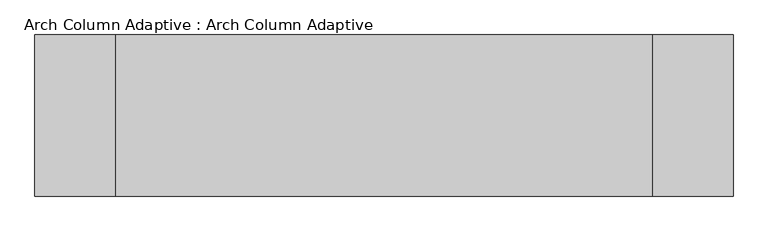
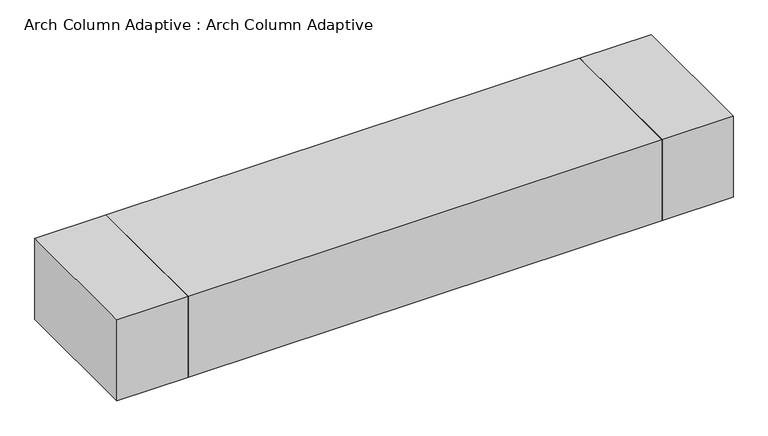
"""IFC4 building model written with IfcOpenShell, lengths in millimetres: proxy geometry, Arch Column Adaptive : Arch Column Adaptive."""

from ifc_helpers import new_model, si_unit, frame, origin, place, context, project, spatial, polyline, outline, extrude, source, transform, mapped, element, save


def arch_column_adaptive_arch_column_adaptive_6fcdb71c(model_context):
    return source(origin(), model_context, "Body", "SweptSolid", [
        extrude(outline(polyline([(5000.0, -1500.0), (5000.0, 1500.0), (6500.0, 1500.0), (6500.0, -1500.0), (5000.0, -1500.0)])), frame((0.0, 0.0, 23611.4), z_axis=(0.0, 0.0, 1.0), x_axis=(1.0, 0.0, 0.0)), (0.0, 0.0, 1.0), 1800.0),
        extrude(outline(polyline([(-5000.0, 1500.0), (-5000.0, -1500.0), (-6500.0, -1500.0), (-6500.0, 1500.0), (-5000.0, 1500.0)])), frame((0.0, 0.0, 23611.4), z_axis=(0.0, 0.0, 1.0), x_axis=(1.0, 0.0, 0.0)), (0.0, 0.0, 1.0), 1800.0),
        extrude(outline(polyline([(-5000.0, -1500.0), (-5000.0, 1500.0), (5000.0, 1500.0), (5000.0, -1500.0), (-5000.0, -1500.0)])), frame((0.0, 0.0, 23611.4), z_axis=(0.0, 0.0, 1.0), x_axis=(1.0, 0.0, 0.0)), (0.0, 0.0, 1.0), 1800.0),
    ])


if __name__ == "__main__":
    model = new_model("IFC4")
    model_context = context("Model", 3, world=origin())
    ifc_project = project(units=[si_unit("LENGTHUNIT", "METRE", prefix="MILLI")], contexts=[model_context])
    site = spatial("IfcSite", under=ifc_project)
    building = spatial("IfcBuilding", under=site)
    placement = place(None, origin())
    arch_column_adaptive_arch_column_adaptive_shape = arch_column_adaptive_arch_column_adaptive_6fcdb71c(model_context)
    element("IfcBuildingElementProxy", 1, Name="Arch Column Adaptive : Arch Column Adaptive", ObjectType="Arch Column Adaptive : Arch Column Adaptive", at=placement, inside=building, context=model_context, shape_type="MappedRepresentation", body=[
        mapped(arch_column_adaptive_arch_column_adaptive_shape, transform((0.0, 0.0, 0.0), x_axis=(1.0, 0.0, 0.0), y_axis=(0.0, 1.0, 0.0), z_axis=(0.0, 0.0, 1.0))),
    ])
    save(model, "model.ifc")

# Revit data of these elements
# Type "Arch Column Adaptive : Arch Column Adaptive"
#   Top Width = 3000 mm
#   Length [instance default] = 21000 mm
#   Height [instance default] = 50000 mm
#   Default Elevation = 0
# Element 1 (IfcBuildingElementProxy, "Arch Column Adaptive : Arch Column Adaptive")
#   Height = 23611.4 mm
